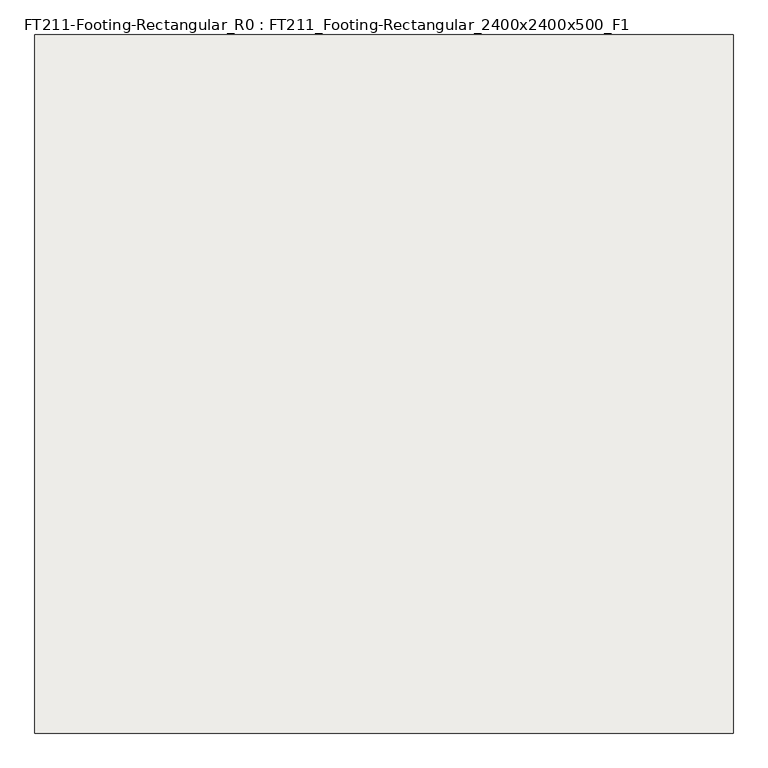
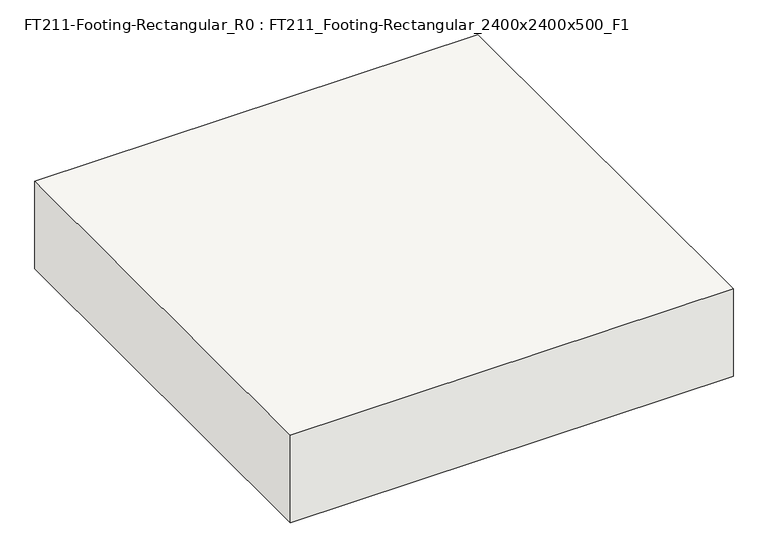
"""IFC4 building model written with IfcOpenShell, lengths in millimetres: slab geometry, FT211-Footing-Rectangular_R0 : FT211_Footing-Rectangular_2400x2400x500_F1."""

import ifcopenshell
import ifcopenshell.guid

model = None  # the IFC model being written
_history = None  # IfcOwnerHistory: only IFC2X3 demands one
_inside = {}  # id of a spatial element -> (the spatial element, [elements in it])
_under = {}  # id of a project, library or spatial element -> (it, [spatial elements below it])
_declared = {}  # id of a project -> (the project, [libraries it declares])
_typed = {}  # id of a type object -> (the type object, [elements of that type])
_made_of = {}  # id of a material, layer set ... -> (it, [elements and type objects made of it])


def new_model(schema):
    """Start an empty IFC model of exactly this schema.

    Asked for "IFC4X3", IfcOpenShell would pick the latest addendum, in which some entities
    have other attributes; the version numbers below select the first issue.
    IFC2X3 requires an IfcOwnerHistory on every rooted entity: one is made here for all.
    """
    global model, _history
    if schema == "IFC4X3":
        model = ifcopenshell.file(schema_version=(4, 3, 0, 0))
    else:
        model = ifcopenshell.file(schema=schema)
    _inside.clear()
    _under.clear()
    _declared.clear()
    _typed.clear()
    _made_of.clear()
    _history = None
    if model.schema == "IFC2X3":
        org = make("IfcOrganization", Name="unknown")
        user = make(
            "IfcPersonAndOrganization",
            ThePerson=make("IfcPerson", FamilyName="unknown"),
            TheOrganization=org,
        )
        app = make(
            "IfcApplication",
            ApplicationDeveloper=org,
            Version="unknown",
            ApplicationFullName="unknown",
            ApplicationIdentifier="unknown",
        )
        _history = make(
            "IfcOwnerHistory",
            OwningUser=user,
            OwningApplication=app,
            ChangeAction="ADDED",
            CreationDate=0,
        )
    return model


def make(cls, **values):
    """One entity of the class cls with the attributes given. An attribute that is None is left unset."""
    return model.create_entity(
        cls, **{name: value for name, value in values.items() if value is not None}
    )


def rooted(cls, **values):
    """An entity with a GlobalId (a new one), such as an element, a storey or a relation."""
    return make(cls, GlobalId=ifcopenshell.guid.new(), OwnerHistory=_history, **values)


def si_unit(unit_type, name, prefix=None):
    """IfcSIUnit, for example si_unit("LENGTHUNIT", "METRE", prefix="MILLI")."""
    return make("IfcSIUnit", UnitType=unit_type, Prefix=prefix, Name=name)


def assignment(units):
    """IfcUnitAssignment: the units of a project."""
    return None if units is None else make("IfcUnitAssignment", Units=units)


def point(xyz):
    """IfcCartesianPoint."""
    return None if xyz is None else make("IfcCartesianPoint", Coordinates=xyz)


def direction(xyz):
    """IfcDirection."""
    return None if xyz is None else make("IfcDirection", DirectionRatios=xyz)


def frame(location, z_axis=None, x_axis=None):
    """IfcAxis2Placement3D, a coordinate frame: its origin and axes. An axis left out is left unset."""
    return make(
        "IfcAxis2Placement3D",
        Location=point(location),
        Axis=direction(z_axis),
        RefDirection=direction(x_axis),
    )


def origin():
    """The frame at (0, 0, 0) with its axes left unset."""
    return frame((0.0, 0.0, 0.0))


def place(relative_to, where):
    """IfcLocalPlacement: puts the frame where relative to a parent placement (None: the world)."""
    return make(
        "IfcLocalPlacement", PlacementRelTo=relative_to, RelativePlacement=where
    )


def context(
    kind, dimensions, precision=None, world=None, true_north=None, identifier=None
):
    """IfcGeometricRepresentationContext, for example the 3D "Model" context."""
    return make(
        "IfcGeometricRepresentationContext",
        ContextIdentifier=identifier,
        ContextType=kind,
        CoordinateSpaceDimension=dimensions,
        Precision=precision,
        WorldCoordinateSystem=world,
        TrueNorth=true_north,
    )


def project(units=None, contexts=None):
    """IfcProject with its units and contexts."""
    return rooted(
        "IfcProject",
        Name="project",
        RepresentationContexts=contexts,
        UnitsInContext=assignment(units),
    )


def spatial(cls, under=None, at=None, **own):
    """A site, building, storey or space (cls), placed at a placement, below another one or the project."""
    s = rooted(cls, ObjectPlacement=at, **own)
    if under is not None:
        _under.setdefault(under.id(), (under, []))[1].append(s)
    return s


def polyline(points):
    """IfcPolyline through the points."""
    return make("IfcPolyline", Points=[point(p) for p in points])


def outline(outer, holes=None, kind="AREA"):
    """IfcArbitraryClosedProfileDef: a profile drawn as a closed curve; with holes, ...WithVoids."""
    if holes is None:
        return make("IfcArbitraryClosedProfileDef", ProfileType=kind, OuterCurve=outer)
    return make(
        "IfcArbitraryProfileDefWithVoids",
        ProfileType=kind,
        OuterCurve=outer,
        InnerCurves=holes,
    )


def extrude(swept, where, along, depth):
    """IfcExtrudedAreaSolid: the profile swept, set in the frame where, extruded along a direction by depth."""
    return make(
        "IfcExtrudedAreaSolid",
        SweptArea=swept,
        Position=where,
        ExtrudedDirection=direction(along),
        Depth=depth,
    )


def shape(context_of_items, identifier, shape_type, items):
    """IfcShapeRepresentation: the items that make up one representation, for example the "Body"."""
    return make(
        "IfcShapeRepresentation",
        ContextOfItems=context_of_items,
        RepresentationIdentifier=identifier,
        RepresentationType=shape_type,
        Items=items,
    )


def source(mapping_origin, context_of_items, identifier, shape_type, items):
    """IfcRepresentationMap: a shape defined once, which mapped items show again and again."""
    return make(
        "IfcRepresentationMap",
        MappingOrigin=mapping_origin,
        MappedRepresentation=shape(context_of_items, identifier, shape_type, items),
    )


def transform(
    local_origin,
    x_axis=None,
    y_axis=None,
    z_axis=None,
    scale=None,
    scale2=None,
    scale3=None,
    uniform=True,
):
    """IfcCartesianTransformationOperator3D, or its non-uniform kind. x_axis, y_axis, z_axis: its Axis1, 2, 3."""
    if uniform:
        return make(
            "IfcCartesianTransformationOperator3D",
            Axis1=direction(x_axis),
            Axis2=direction(y_axis),
            LocalOrigin=point(local_origin),
            Scale=scale,
            Axis3=direction(z_axis),
        )
    return make(
        "IfcCartesianTransformationOperator3DnonUniform",
        Axis1=direction(x_axis),
        Axis2=direction(y_axis),
        LocalOrigin=point(local_origin),
        Scale=scale,
        Axis3=direction(z_axis),
        Scale2=scale2,
        Scale3=scale3,
    )


def mapped(mapping_source, mapping_target):
    """IfcMappedItem: shows the shape of a source again, moved by a transform."""
    return make(
        "IfcMappedItem", MappingSource=mapping_source, MappingTarget=mapping_target
    )


def made_of(thing, what):
    """Note that an element or type object is made of a material, layer set ...; save() writes the relation."""
    if what is not None:
        _made_of.setdefault(what.id(), (what, []))[1].append(thing)
    return thing


def element(
    cls,
    number,
    at=None,
    inside=None,
    cuts=None,
    type_object=None,
    material=None,
    context=None,
    identifier="Body",
    shape_type=None,
    held_by="IfcProductDefinitionShape",
    body=None,
    shapes=None,
    **own,
):
    """One element of the class cls, such as IfcWall. Its Tag is "e" and its number.

    at: its placement. inside: the storey or other place that contains it. cuts: it is an
    opening in that element (IfcRelVoidsElement). A single representation is given by context,
    identifier, shape_type and body (its items); several are given by shapes. held_by: the class
    of the entity that holds the representations. save() writes the other relations.
    """
    e = rooted(cls, Tag="e%d" % number, ObjectPlacement=at, **own)
    if body is not None:
        shapes = [shape(context, identifier, shape_type, body)]
    if shapes is not None:
        e.Representation = make(held_by, Representations=shapes)
    if inside is not None:
        _inside.setdefault(inside.id(), (inside, []))[1].append(e)
    if cuts is not None:
        rooted(
            "IfcRelVoidsElement", RelatingBuildingElement=cuts, RelatedOpeningElement=e
        )
    if type_object is not None:
        _typed.setdefault(type_object.id(), (type_object, []))[1].append(e)
    return made_of(e, material)


def aggregate(whole, parts):
    """IfcRelAggregates: a whole, such as a stair, and the parts it consists of."""
    return rooted("IfcRelAggregates", RelatingObject=whole, RelatedObjects=parts)


def save(model, path):
    """Write the relations noted so far, then the file.

    IfcRelAggregates (storeys below a building ...), IfcRelContainedInSpatialStructure (elements
    in a storey), IfcRelDefinesByType, IfcRelAssociatesMaterial and IfcRelDeclares: one each for
    every whole, place, type object, material and project.
    """
    for whole, parts in _under.values():
        aggregate(whole, parts)
    for where, things in _inside.values():
        rooted(
            "IfcRelContainedInSpatialStructure",
            RelatedElements=things,
            RelatingStructure=where,
        )
    for kind, things in _typed.values():
        rooted("IfcRelDefinesByType", RelatedObjects=things, RelatingType=kind)
    for what, things in _made_of.values():
        rooted("IfcRelAssociatesMaterial", RelatedObjects=things, RelatingMaterial=what)
    for by, libraries in _declared.values():
        rooted("IfcRelDeclares", RelatingContext=by, RelatedDefinitions=libraries)
    model.write(path)


def ft211_footing_rectangular_r0_ft211_footing_rectangular_5fe39465(model_context):
    return source(origin(), model_context, "Body", "SweptSolid", [
        extrude(outline(polyline([(1200.0, 1200.0), (1200.0, -1200.0), (-1200.0, -1200.0), (-1200.0, 1200.0), (1200.0, 1200.0)])), frame((0.0, 0.0, -500.0), z_axis=(0.0, 0.0, 1.0), x_axis=(1.0, 0.0, 0.0)), (0.0, 0.0, 1.0), 500.0),
    ])


if __name__ == "__main__":
    model = new_model("IFC4")
    model_context = context("Model", 3, world=origin())
    ifc_project = project(units=[si_unit("LENGTHUNIT", "METRE", prefix="MILLI")], contexts=[model_context])
    site = spatial("IfcSite", under=ifc_project)
    building = spatial("IfcBuilding", under=site)
    placement = place(None, origin())
    ft211_footing_rectangular_r0_ft211_footing_rectangular_shape = ft211_footing_rectangular_r0_ft211_footing_rectangular_5fe39465(model_context)
    element("IfcSlab", 1, ObjectType="FT211-Footing-Rectangular_R0 : FT211_Footing-Rectangular_2400x2400x500_F1", at=placement, inside=building, context=model_context, shape_type="MappedRepresentation", body=[
        mapped(ft211_footing_rectangular_r0_ft211_footing_rectangular_shape, transform((0.0, 0.0, 0.0), x_axis=(1.0, 0.0, 0.0), y_axis=(0.0, 1.0, 0.0), z_axis=(0.0, 0.0, 1.0))),
    ])
    save(model, "model.ifc")

# Revit data of these elements
# Type "FT211-Footing-Rectangular_R0 : FT211_Footing-Rectangular_2400x2400x500_F1"
#   Top bar = "D25@300"
#   Description = "UG Shallow Foundation"
#   Bottom bar = "D20@300"
#   Width = 2400 mm
#   Length = 2400 mm
#   Foundation Thickness = 500 mm
#   Structural Material [instance default] = A03AC032-00007_Structural Concrete_Type1_25MPa-30Mpa
#   Assembly Code = ""
# Element 1 (IfcSlab, "FT211-Footing-Rectangular_R0 : FT211_Footing-Rectangular_2400x2400x500_F1")
#   Materials on its faces: "A03AC032-00007_Structural Concrete_Type1_25MPa-30Mpa"
# Materials
#   "A03AC032-00007_Structural Concrete_Type1_25MPa-30Mpa": class "Concrete", colour RGB 176 176 176, transparency 0, Keynote = "09910.A1", Description = "Reinf. Conc.", W00) Work Master Code = "A03AC032-00007", W01) Work Master_Lv1 = "Concrete Work", W02) Work Master_Lv2 = "Substructure Work", W03) Work Master_Spec.1 = "Structural Concrete", W04) Work Master_Spec.2 = "Cement Type-1", W05) Work Master_Spec.3 = "25MPa < F'c (Cylinder Strength) ≤ 30MPa", Cost = 0
